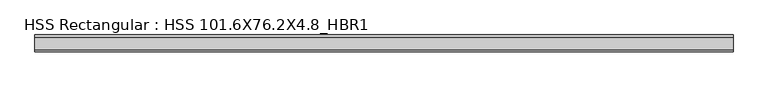
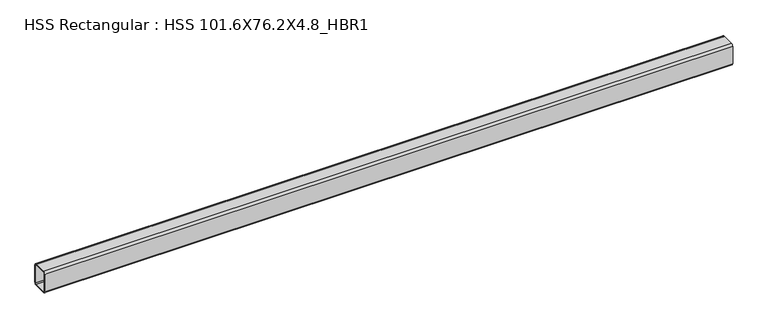
"""IFC4 building model written with IfcOpenShell, lengths in millimetres: beam geometry, HSS Rectangular : HSS 101.6X76.2X4.8_HBR1."""

from ifc_helpers import new_model, si_unit, point, frame, frame_2d, origin, place, context, project, spatial, polyline, circle_curve, trimmed, segment, composite_curve, outline, extrude, source, transform, mapped, element, save


def hss_rectangular_hss_101_6x76_2x4_8_hbr1_afe8bef4(model_context):
    return source(origin(), model_context, "Body", "SweptSolid", [
        extrude(outline(composite_curve([segment(polyline([(38.1, 41.275), (38.1, -41.275)]), True, "CONTINUOUS"), segment(trimmed(circle_curve(frame_2d((28.575, -41.275)), 9.525), [point((38.1, -41.275))], [point((28.575, -50.8))], False, "CARTESIAN"), True, "CONTINUOUS"), segment(polyline([(28.575, -50.8), (-28.575, -50.8)]), True, "CONTINUOUS"), segment(trimmed(circle_curve(frame_2d((-28.575, -41.275)), 9.525), [point((-28.575, -50.8))], [point((-38.1, -41.275))], False, "CARTESIAN"), True, "CONTINUOUS"), segment(polyline([(-38.1, -41.275), (-38.1, 41.275)]), True, "CONTINUOUS"), segment(trimmed(circle_curve(frame_2d((-28.575, 41.275)), 9.525), [point((-38.1, 41.275))], [point((-28.575, 50.8))], False, "CARTESIAN"), True, "CONTINUOUS"), segment(polyline([(-28.575, 50.8), (28.575, 50.8)]), True, "CONTINUOUS"), segment(trimmed(circle_curve(frame_2d((28.575, 41.275)), 9.525), [point((28.575, 50.8))], [point((38.1, 41.275))], False, "CARTESIAN"), True, "CONTINUOUS")], self_intersect=False), holes=[composite_curve([segment(trimmed(circle_curve(frame_2d((-28.575, 41.275)), 4.7625), [point((-28.575, 46.0375))], [point((-33.3375, 41.275))], True, "CARTESIAN"), True, "CONTINUOUS"), segment(polyline([(-33.3375, 41.275), (-33.3375, -41.275)]), True, "CONTINUOUS"), segment(trimmed(circle_curve(frame_2d((-28.575, -41.275)), 4.7625), [point((-33.3375, -41.275))], [point((-28.575, -46.0375))], True, "CARTESIAN"), True, "CONTINUOUS"), segment(polyline([(-28.575, -46.0375), (28.575, -46.0375)]), True, "CONTINUOUS"), segment(trimmed(circle_curve(frame_2d((28.575, -41.275)), 4.7625), [point((28.575, -46.0375))], [point((33.3375, -41.275))], True, "CARTESIAN"), True, "CONTINUOUS"), segment(polyline([(33.3375, -41.275), (33.3375, 41.275)]), True, "CONTINUOUS"), segment(trimmed(circle_curve(frame_2d((28.575, 41.275)), 4.7625), [point((33.3375, 41.275))], [point((28.575, 46.0375))], True, "CARTESIAN"), True, "CONTINUOUS"), segment(polyline([(28.575, 46.0375), (-28.575, 46.0375)]), True, "CONTINUOUS")], self_intersect=False)]), frame((-1490.7588751, 0.0, 0.0), z_axis=(1.0, 0.0, 0.0), x_axis=(0.0, 1.0, 0.0)), (0.0, 0.0, 1.0), 3136.010921),
    ])


if __name__ == "__main__":
    model = new_model("IFC4")
    model_context = context("Model", 3, world=origin())
    ifc_project = project(units=[si_unit("LENGTHUNIT", "METRE", prefix="MILLI")], contexts=[model_context])
    site = spatial("IfcSite", under=ifc_project)
    building = spatial("IfcBuilding", under=site)
    placement = place(None, origin())
    hss_rectangular_hss_101_6x76_2x4_8_hbr1_shape = hss_rectangular_hss_101_6x76_2x4_8_hbr1_afe8bef4(model_context)
    element("IfcBeam", 1, ObjectType="HSS Rectangular : HSS 101.6X76.2X4.8_HBR1", at=placement, inside=building, context=model_context, shape_type="MappedRepresentation", body=[
        mapped(hss_rectangular_hss_101_6x76_2x4_8_hbr1_shape, transform((0.0, 0.0, 0.0), x_axis=(1.0, 0.0, 0.0), y_axis=(0.0, 1.0, 0.0), z_axis=(0.0, 0.0, 1.0))),
    ])
    save(model, "model.ifc")

# Revit data of these elements
# Type "HSS Rectangular : HSS 101.6X76.2X4.8_HBR1"
#   Section Name Key = "HSS 4X3X3/16"
#   Assembly Code = "B10"
#   Width = 7.62 cm
#   Wall Nominal Thickness = 0.4763 cm
#   Wall Design Thickness = 0.442 cm
#   Torsional Moment of Inertia = 260.561 cm⁴
#   Torsional Modulus = 61.2876 cm³
#   Section Area = 14.4516 cm²
#   Plastic Modulus weak axis = 40.3122 cm³
#   Plastic Modulus strong axis = 49.1612 cm³
#   Perimeter = 0.881482 m²/m
#   Outer Fillet = 0.9525 cm
#   Nominal Weight = 12.1285 kgf/m
#   Moment of Inertia weak axis = 131.529 cm⁴
#   Moment of Inertia strong axis = 205.202 cm⁴
#   Inner Fillet = 0.4763 cm
#   Height = 10.16 cm
#   Elastic Modulus weak axis = 34.4128 cm³
#   Elastic Modulus strong axis = 40.476 cm³
#   Centroid Vertical = 5.08 cm
#   Centroid Horizontal = 3.81 cm
#   Length [instance default] = 1524 mm
#   Structural Material [instance default] = Steel ASTM A500, Grade B, Rectangular and Square
#   Principal Axes Angle = 0
# Element 1 (IfcBeam, "HSS Rectangular : HSS 101.6X76.2X4.8_HBR1")
#   Structural Material = Steel ASTM A992
#   Materials on its faces: "Steel ASTM A992"
# Materials
#   "Steel ASTM A500, Grade B, Rectangular and Square": class "Metal", colour RGB 199 199 199, transparency 0, Description = "Carbon steel", Cost = 0
#   "Steel ASTM A992": class "Metal", colour RGB 199 199 199, transparency 0, Description = "Structural steel 50ksi", Cost = 0
